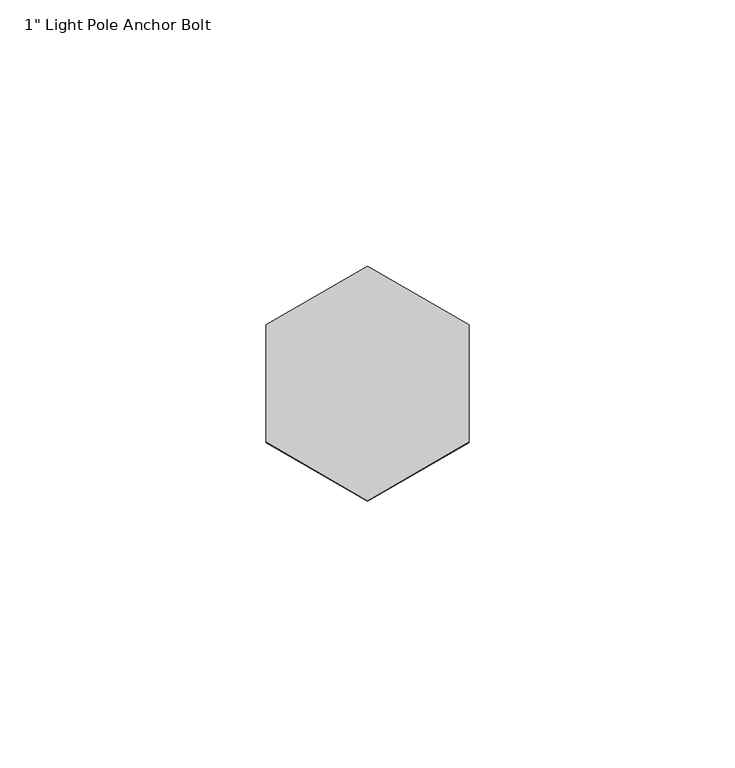
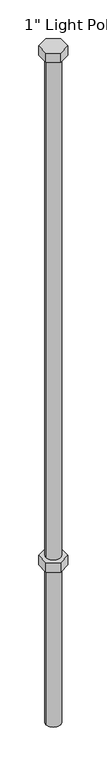
"""IFC4 building model written with IfcOpenShell, lengths in millimetres: proxy geometry."""

from ifc_helpers import new_model, si_unit, point, frame, origin, origin_with_axes, origin_2d, place, context, project, spatial, polyline, circle_curve, trimmed, segment, composite_curve, outline, extrude, source, transform, mapped, element, save


def proxy_fbbee035(model_context):
    return source(origin(), model_context, "Body", "SweptSolid", [
        extrude(outline(polyline([(-19.05, 10.9985226), (0.0, 21.9970453), (19.05, 10.9985226), (19.05, -10.9985226), (0.0, -21.9970453), (-19.05, -10.9985226), (-19.05, 10.9985226)])), frame((0.0, 0.0, -931.465625), z_axis=(0.0, 0.0, 1.0), x_axis=(1.0, 0.0, 0.0)), (0.0, 0.0, 1.0), 17.065625),
        extrude(outline(polyline([(-19.05, -10.9985226), (-19.05, 10.9985226), (0.0, 21.9970453), (19.05, 10.9985226), (19.05, -10.9985226), (0.0, -21.9970453), (-19.05, -10.9985226)])), origin_with_axes(), (0.0, 0.0, 1.0), 17.065625),
        extrude(outline(composite_curve([segment(trimmed(circle_curve(origin_2d(), 12.7), [point((-12.7, 0.0))], [point((12.7, 0.0))], False, "CARTESIAN"), True, "CONTINUOUS"), segment(trimmed(circle_curve(origin_2d(), 12.7), [point((12.7, 0.0))], [point((-12.7, 0.0))], False, "CARTESIAN"), True, "CONTINUOUS")], self_intersect=False)), frame((0.0, 0.0, -1219.2), z_axis=(0.0, 0.0, 1.0), x_axis=(1.0, 0.0, 0.0)), (0.0, 0.0, 1.0), 1219.2),
    ])


if __name__ == "__main__":
    model = new_model("IFC4")
    model_context = context("Model", 3, world=origin())
    ifc_project = project(units=[si_unit("LENGTHUNIT", "METRE", prefix="MILLI")], contexts=[model_context])
    site = spatial("IfcSite", under=ifc_project)
    building = spatial("IfcBuilding", under=site)
    placement = place(None, origin())
    proxy_shape = proxy_fbbee035(model_context)
    element("IfcBuildingElementProxy", 1, Name="050523 - W_P_C - Fastenings - Lag Bolt or Thru Bolt : 1\" Light Pole Anchor Bolt", ObjectType="050523 - W_P_C - Fastenings - Lag Bolt or Thru Bolt : 1\" Light Pole Anchor Bolt", at=placement, inside=building, context=model_context, shape_type="MappedRepresentation", body=[
        mapped(proxy_shape, transform((0.0, 0.0, 0.0), x_axis=(1.0, 0.0, 0.0), y_axis=(0.0, 1.0, 0.0), z_axis=(0.0, 0.0, 1.0))),
    ])
    save(model, "model.ifc")

# Revit data of these elements
# Type "050523 - W_P_C - Fastenings - Lag Bolt or Thru Bolt : 1\" Light Pole Anchor Bolt"
#   Thickness_of_Substrate [instance default] = 0' - 1"
#   Side = 0' - 0 111/128"
#   Radius = 0' - 0 1/2"
#   Length = 4' - 0"
#   Head Size = 0' - 1 1/2"
#   Head Radius = 0' - 0 3/4"
#   Head Height = 0' - 0 43/64"
#   Diameter = 0' - 1"
#   Default Elevation = 4' - 0"
#   Nut_Visibility [instance default] = yes
#   Bolt Material (Size) [instance default] = 5/8" GALV. ANCHOR BOLT @ 24" O.C. (6" MIN. EMBEDMENT)
# Element 1 (IfcBuildingElementProxy, "050523 - W_P_C - Fastenings - Lag Bolt or Thru Bolt : 1\" Light Pole Anchor Bolt")
#   Thickness_of_Substrate = 3' - 0"
#   Bolt Material (Size) = STRUCTURAL BOLTS (PAINT TO MATCH STEEL FINISH)
#   Materials on its faces: "STRUCTURAL BOLTS (PAINT TO MATCH STEEL FINISH)"
# Materials
#   "5/8\" GALV. ANCHOR BOLT @ 24\" O.C. (6\" MIN. EMBEDMENT)": class "Generic", colour RGB 120 120 120, transparency 0, Cost = 0
#   "STRUCTURAL BOLTS (PAINT TO MATCH STEEL FINISH)": class "Generic", colour RGB 120 120 120, transparency 0, Cost = 0
